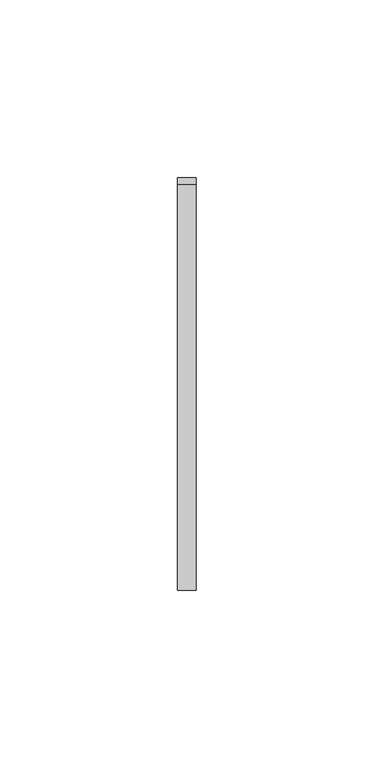
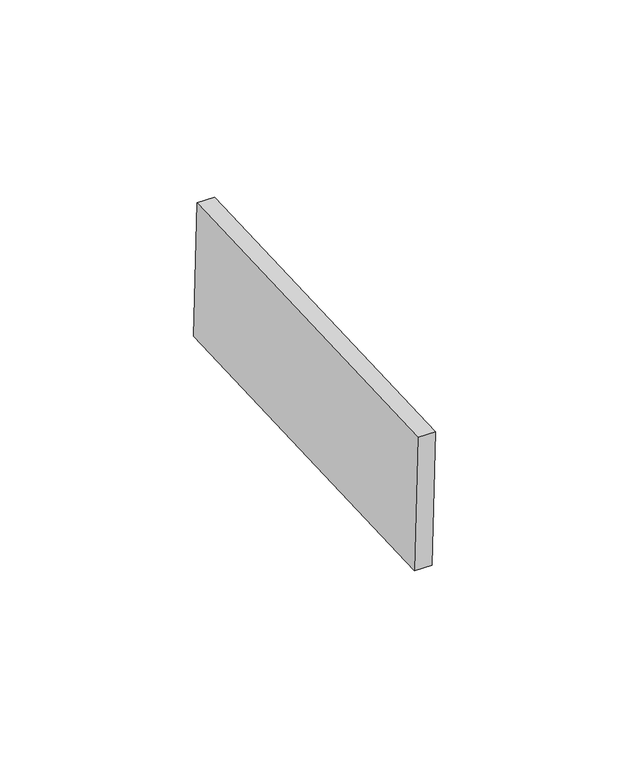
"""IFC4 building model written with IfcOpenShell, lengths in millimetres: proxy geometry, Inner panel:Inner panel:1:Inner panel:1 : Inner panel:Inner panel:300324:2:Inner panel:1:Inner panel:1 : Inner panel:Inner panel:300324:2 : Inner panel:Inner panel:1:Inner panel:1 : Inner panel:Inner panel:300324:300043:88 : Inner panel:Inner panel:1:Inner panel:1 : Inner panel:Inner panel:300324:2:Inner panel:1:Inner panel:1 : Inner panel:Inner panel:300324:2 : Inner panel:Inner panel:1:Inner panel:1 : Inner panel:Inner panel:300324:300043:308120."""

from ifc_helpers import new_model, si_unit, frame, origin, place, context, project, spatial, polyline, outline, extrude, source, transform, mapped, element, save


def generic_models_1fb866dc(model_context):
    return source(origin(), model_context, "Body", "SweptSolid", [
        extrude(outline(polyline([(0.0, -114.2999999), (0.0, 0.0), (5.2138089, 0.0), (5.2138089, -114.2999999), (0.0, -114.2999999)])), frame((593123.795117, -568168.273882, 8806.9397902), z_axis=(0.0, -0.04163054471215927, 0.9991330730923529), x_axis=(-1.0, 0.0, 0.0)), (0.0, 0.0, 1.0), 43.2233908),
    ])


if __name__ == "__main__":
    model = new_model("IFC4")
    model_context = context("Model", 3, world=origin())
    ifc_project = project(units=[si_unit("LENGTHUNIT", "METRE", prefix="MILLI")], contexts=[model_context])
    site = spatial("IfcSite", under=ifc_project)
    building = spatial("IfcBuilding", under=site)
    placement = place(None, origin())
    generic_models_shape = generic_models_1fb866dc(model_context)
    element("IfcBuildingElementProxy", 1, Name="Inner panel:Inner panel:1:Inner panel:1 : Inner panel:Inner panel:300324:2:Inner panel:1:Inner panel:1 : Inner panel:Inner panel:300324:2 : Inner panel:Inner panel:1:Inner panel:1 : Inner panel:Inner panel:300324:300043:88 : Inner panel:Inner panel:1:Inner panel:1 : Inner panel:Inner panel:300324:2:Inner panel:1:Inner panel:1 : Inner panel:Inner panel:300324:2 : Inner panel:Inner panel:1:Inner panel:1 : Inner panel:Inner panel:300324:300043:308120", ObjectType="Inner panel:Inner panel:1:Inner panel:1 : Inner panel:Inner panel:300324:2:Inner panel:1:Inner panel:1 : Inner panel:Inner panel:300324:2 : Inner panel:Inner panel:1:Inner panel:1 : Inner panel:Inner panel:300324:300043:88 : Inner panel:Inner panel:1:Inner panel:1 : Inner panel:Inner panel:300324:2:Inner panel:1:Inner panel:1 : Inner panel:Inner panel:300324:2 : Inner panel:Inner panel:1:Inner panel:1 : Inner panel:Inner panel:300324:300043:308120", at=placement, inside=building, context=model_context, shape_type="MappedRepresentation", body=[
        mapped(generic_models_shape, transform((0.0, 0.0, 0.0), x_axis=(1.0, 0.0, 0.0), y_axis=(0.0, 1.0, 0.0), z_axis=(0.0, 0.0, 1.0))),
    ])
    save(model, "model.ifc")

# Revit data of these elements
# Type "Inner panel:Inner panel:1:Inner panel:1 : Inner panel:Inner panel:300324:2:Inner panel:1:Inner panel:1 : Inner panel:Inner panel:300324:2 : Inner panel:Inner panel:1:Inner panel:1 : Inner panel:Inner panel:300324:300043:88 : Inner panel:Inner panel:1:Inner panel:1 : Inner panel:Inner panel:300324:2:Inner panel:1:Inner panel:1 : Inner panel:Inner panel:300324:2 : Inner panel:Inner panel:1:Inner panel:1 : Inner panel:Inner panel:300324:300043:308120"
#   NameOverride = "Inner panel:Inner panel:1:Inner panel:1 : Inner panel:Inner panel:300324:2:Inner panel:1:Inner panel:1 : Inner panel:Inner panel:300324:2 : Inner panel:Inner panel:1:Inner panel:1 : Inner panel:Inner panel:300324:300043:308120"
#   ObjectTypeOverride = "Inner panel:1:Inner panel:1 : Inner panel:Inner panel:300324:2 : Inner panel:Inner panel:1:Inner panel:1 : Inner panel:Inner panel:300324:300043"
#   Reference = "Inner panel"
#   Tag = "308120"
# Element 1 (IfcBuildingElementProxy, "Inner panel:Inner panel:1:Inner panel:1 : Inner panel:Inner panel:300324:2:Inner panel:1:Inner panel:1 : Inner panel:Inner panel:300324:2 : Inner panel:Inner panel:1:Inner panel:1 : Inner panel:Inner panel:300324:300043:88 : Inner panel:Inner panel:1:Inner panel:1 : Inner panel:Inner panel:300324:2:Inner panel:1:Inner panel:1 : Inner panel:Inner panel:300324:2 : Inner panel:Inner panel:1:Inner panel:1 : Inner panel:Inner panel:300324:300043:308120")
#   Materials on its faces: "SLIDING CLIP"
# Materials
#   "SLIDING CLIP": class "Generic", colour RGB 120 120 120, transparency 0, Cost = 0
